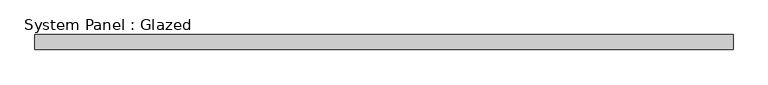
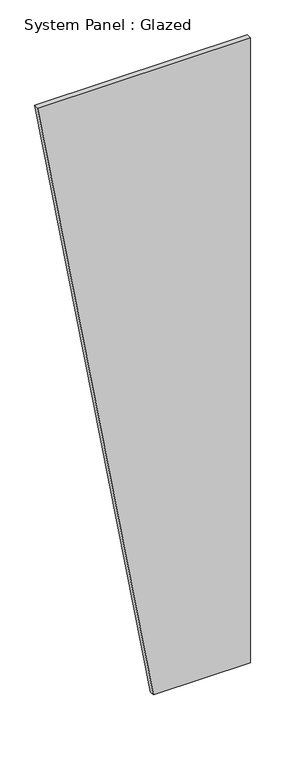
"""IFC4 building model written with IfcOpenShell, lengths in millimetres: plate geometry, System Panel : Glazed."""

import ifcopenshell
import ifcopenshell.guid

model = None  # the IFC model being written
_history = None  # IfcOwnerHistory: only IFC2X3 demands one
_inside = {}  # id of a spatial element -> (the spatial element, [elements in it])
_under = {}  # id of a project, library or spatial element -> (it, [spatial elements below it])
_declared = {}  # id of a project -> (the project, [libraries it declares])
_typed = {}  # id of a type object -> (the type object, [elements of that type])
_made_of = {}  # id of a material, layer set ... -> (it, [elements and type objects made of it])


def new_model(schema):
    """Start an empty IFC model of exactly this schema.

    Asked for "IFC4X3", IfcOpenShell would pick the latest addendum, in which some entities
    have other attributes; the version numbers below select the first issue.
    IFC2X3 requires an IfcOwnerHistory on every rooted entity: one is made here for all.
    """
    global model, _history
    if schema == "IFC4X3":
        model = ifcopenshell.file(schema_version=(4, 3, 0, 0))
    else:
        model = ifcopenshell.file(schema=schema)
    _inside.clear()
    _under.clear()
    _declared.clear()
    _typed.clear()
    _made_of.clear()
    _history = None
    if model.schema == "IFC2X3":
        org = make("IfcOrganization", Name="unknown")
        user = make(
            "IfcPersonAndOrganization",
            ThePerson=make("IfcPerson", FamilyName="unknown"),
            TheOrganization=org,
        )
        app = make(
            "IfcApplication",
            ApplicationDeveloper=org,
            Version="unknown",
            ApplicationFullName="unknown",
            ApplicationIdentifier="unknown",
        )
        _history = make(
            "IfcOwnerHistory",
            OwningUser=user,
            OwningApplication=app,
            ChangeAction="ADDED",
            CreationDate=0,
        )
    return model


def make(cls, **values):
    """One entity of the class cls with the attributes given. An attribute that is None is left unset."""
    return model.create_entity(
        cls, **{name: value for name, value in values.items() if value is not None}
    )


def rooted(cls, **values):
    """An entity with a GlobalId (a new one), such as an element, a storey or a relation."""
    return make(cls, GlobalId=ifcopenshell.guid.new(), OwnerHistory=_history, **values)


def si_unit(unit_type, name, prefix=None):
    """IfcSIUnit, for example si_unit("LENGTHUNIT", "METRE", prefix="MILLI")."""
    return make("IfcSIUnit", UnitType=unit_type, Prefix=prefix, Name=name)


def assignment(units):
    """IfcUnitAssignment: the units of a project."""
    return None if units is None else make("IfcUnitAssignment", Units=units)


def point(xyz):
    """IfcCartesianPoint."""
    return None if xyz is None else make("IfcCartesianPoint", Coordinates=xyz)


def direction(xyz):
    """IfcDirection."""
    return None if xyz is None else make("IfcDirection", DirectionRatios=xyz)


def frame(location, z_axis=None, x_axis=None):
    """IfcAxis2Placement3D, a coordinate frame: its origin and axes. An axis left out is left unset."""
    return make(
        "IfcAxis2Placement3D",
        Location=point(location),
        Axis=direction(z_axis),
        RefDirection=direction(x_axis),
    )


def origin():
    """The frame at (0, 0, 0) with its axes left unset."""
    return frame((0.0, 0.0, 0.0))


def place(relative_to, where):
    """IfcLocalPlacement: puts the frame where relative to a parent placement (None: the world)."""
    return make(
        "IfcLocalPlacement", PlacementRelTo=relative_to, RelativePlacement=where
    )


def context(
    kind, dimensions, precision=None, world=None, true_north=None, identifier=None
):
    """IfcGeometricRepresentationContext, for example the 3D "Model" context."""
    return make(
        "IfcGeometricRepresentationContext",
        ContextIdentifier=identifier,
        ContextType=kind,
        CoordinateSpaceDimension=dimensions,
        Precision=precision,
        WorldCoordinateSystem=world,
        TrueNorth=true_north,
    )


def project(units=None, contexts=None):
    """IfcProject with its units and contexts."""
    return rooted(
        "IfcProject",
        Name="project",
        RepresentationContexts=contexts,
        UnitsInContext=assignment(units),
    )


def spatial(cls, under=None, at=None, **own):
    """A site, building, storey or space (cls), placed at a placement, below another one or the project."""
    s = rooted(cls, ObjectPlacement=at, **own)
    if under is not None:
        _under.setdefault(under.id(), (under, []))[1].append(s)
    return s


def polyline(points):
    """IfcPolyline through the points."""
    return make("IfcPolyline", Points=[point(p) for p in points])


def outline(outer, holes=None, kind="AREA"):
    """IfcArbitraryClosedProfileDef: a profile drawn as a closed curve; with holes, ...WithVoids."""
    if holes is None:
        return make("IfcArbitraryClosedProfileDef", ProfileType=kind, OuterCurve=outer)
    return make(
        "IfcArbitraryProfileDefWithVoids",
        ProfileType=kind,
        OuterCurve=outer,
        InnerCurves=holes,
    )


def extrude(swept, where, along, depth):
    """IfcExtrudedAreaSolid: the profile swept, set in the frame where, extruded along a direction by depth."""
    return make(
        "IfcExtrudedAreaSolid",
        SweptArea=swept,
        Position=where,
        ExtrudedDirection=direction(along),
        Depth=depth,
    )


def shape(context_of_items, identifier, shape_type, items):
    """IfcShapeRepresentation: the items that make up one representation, for example the "Body"."""
    return make(
        "IfcShapeRepresentation",
        ContextOfItems=context_of_items,
        RepresentationIdentifier=identifier,
        RepresentationType=shape_type,
        Items=items,
    )


def source(mapping_origin, context_of_items, identifier, shape_type, items):
    """IfcRepresentationMap: a shape defined once, which mapped items show again and again."""
    return make(
        "IfcRepresentationMap",
        MappingOrigin=mapping_origin,
        MappedRepresentation=shape(context_of_items, identifier, shape_type, items),
    )


def transform(
    local_origin,
    x_axis=None,
    y_axis=None,
    z_axis=None,
    scale=None,
    scale2=None,
    scale3=None,
    uniform=True,
):
    """IfcCartesianTransformationOperator3D, or its non-uniform kind. x_axis, y_axis, z_axis: its Axis1, 2, 3."""
    if uniform:
        return make(
            "IfcCartesianTransformationOperator3D",
            Axis1=direction(x_axis),
            Axis2=direction(y_axis),
            LocalOrigin=point(local_origin),
            Scale=scale,
            Axis3=direction(z_axis),
        )
    return make(
        "IfcCartesianTransformationOperator3DnonUniform",
        Axis1=direction(x_axis),
        Axis2=direction(y_axis),
        LocalOrigin=point(local_origin),
        Scale=scale,
        Axis3=direction(z_axis),
        Scale2=scale2,
        Scale3=scale3,
    )


def mapped(mapping_source, mapping_target):
    """IfcMappedItem: shows the shape of a source again, moved by a transform."""
    return make(
        "IfcMappedItem", MappingSource=mapping_source, MappingTarget=mapping_target
    )


def made_of(thing, what):
    """Note that an element or type object is made of a material, layer set ...; save() writes the relation."""
    if what is not None:
        _made_of.setdefault(what.id(), (what, []))[1].append(thing)
    return thing


def element(
    cls,
    number,
    at=None,
    inside=None,
    cuts=None,
    type_object=None,
    material=None,
    context=None,
    identifier="Body",
    shape_type=None,
    held_by="IfcProductDefinitionShape",
    body=None,
    shapes=None,
    **own,
):
    """One element of the class cls, such as IfcWall. Its Tag is "e" and its number.

    at: its placement. inside: the storey or other place that contains it. cuts: it is an
    opening in that element (IfcRelVoidsElement). A single representation is given by context,
    identifier, shape_type and body (its items); several are given by shapes. held_by: the class
    of the entity that holds the representations. save() writes the other relations.
    """
    e = rooted(cls, Tag="e%d" % number, ObjectPlacement=at, **own)
    if body is not None:
        shapes = [shape(context, identifier, shape_type, body)]
    if shapes is not None:
        e.Representation = make(held_by, Representations=shapes)
    if inside is not None:
        _inside.setdefault(inside.id(), (inside, []))[1].append(e)
    if cuts is not None:
        rooted(
            "IfcRelVoidsElement", RelatingBuildingElement=cuts, RelatedOpeningElement=e
        )
    if type_object is not None:
        _typed.setdefault(type_object.id(), (type_object, []))[1].append(e)
    return made_of(e, material)


def aggregate(whole, parts):
    """IfcRelAggregates: a whole, such as a stair, and the parts it consists of."""
    return rooted("IfcRelAggregates", RelatingObject=whole, RelatedObjects=parts)


def save(model, path):
    """Write the relations noted so far, then the file.

    IfcRelAggregates (storeys below a building ...), IfcRelContainedInSpatialStructure (elements
    in a storey), IfcRelDefinesByType, IfcRelAssociatesMaterial and IfcRelDeclares: one each for
    every whole, place, type object, material and project.
    """
    for whole, parts in _under.values():
        aggregate(whole, parts)
    for where, things in _inside.values():
        rooted(
            "IfcRelContainedInSpatialStructure",
            RelatedElements=things,
            RelatingStructure=where,
        )
    for kind, things in _typed.values():
        rooted("IfcRelDefinesByType", RelatedObjects=things, RelatingType=kind)
    for what, things in _made_of.values():
        rooted("IfcRelAssociatesMaterial", RelatedObjects=things, RelatingMaterial=what)
    for by, libraries in _declared.values():
        rooted("IfcRelDeclares", RelatingContext=by, RelatedDefinitions=libraries)
    model.write(path)


def system_panel_glazed_bcd6892e(model_context):
    return source(origin(), model_context, "Body", "SweptSolid", [
        extrude(outline(polyline([(0.0, 53.0003468), (0.0, 589.4790509), (3657.6, 589.4790509), (3657.6, -589.4790509), (0.0, 53.0003468)])), frame((0.0, -44.45, 0.0), z_axis=(0.0, 1.0, 0.0), x_axis=(0.0, 0.0, 1.0)), (0.0, 0.0, 1.0), 25.4),
    ])


if __name__ == "__main__":
    model = new_model("IFC4")
    model_context = context("Model", 3, world=origin())
    ifc_project = project(units=[si_unit("LENGTHUNIT", "METRE", prefix="MILLI")], contexts=[model_context])
    site = spatial("IfcSite", under=ifc_project)
    building = spatial("IfcBuilding", under=site)
    placement = place(None, origin())
    system_panel_glazed_shape = system_panel_glazed_bcd6892e(model_context)
    element("IfcPlate", 1, ObjectType="System Panel : Glazed", at=placement, inside=building, context=model_context, shape_type="MappedRepresentation", body=[
        mapped(system_panel_glazed_shape, transform((0.0, 0.0, 0.0), x_axis=(1.0, 0.0, 0.0), y_axis=(0.0, 1.0, 0.0), z_axis=(0.0, 0.0, 1.0))),
    ])
    save(model, "model.ifc")

# Revit data of these elements
# Type "System Panel : Glazed"
#   Construction Type Id = "GSP4R"
#   Analytic Construction = "1/8 in Pilkington single glazing"
#   Visual Light Transmittance = 0.9
#   Solar Heat Gain Coefficient = 0.86
#   Heat Transfer Coefficient (U) = 1.18115 BTU/(h·ft²·°F)
#   Define Thermal Properties by = 1
# Element 1 (IfcPlate, "System Panel : Glazed")
#   Materials on its faces: "Glass"
# Materials
#   "Glass": class "Glass", colour RGB 0 128 192, transparency 0.75, Description = "Soda Lime Glass", Cost = 0
